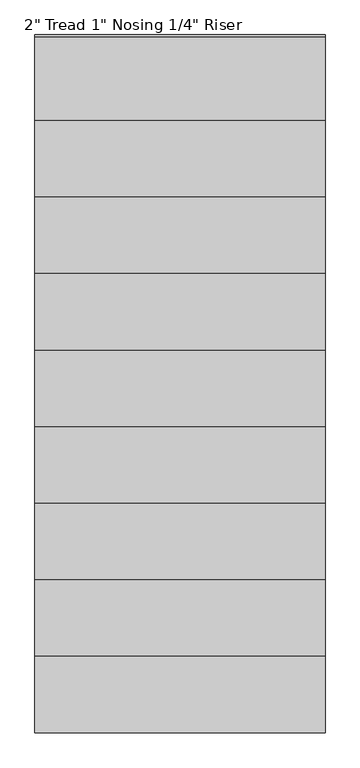
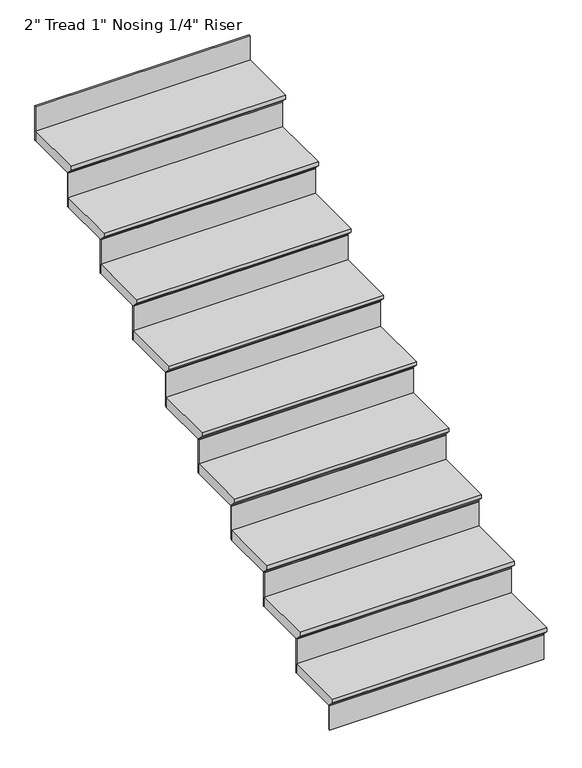
"""IFC4 building model written with IfcOpenShell, lengths in millimetres: stair flight geometry."""

from ifc_helpers import new_model, si_unit, frame, origin, place, context, project, spatial, polyline, outline, extrude, source, transform, mapped, element, save


def stair_flight_2c35b375(model_context):
    return source(origin(), model_context, "Body", "SweptSolid", [
        extrude(outline(polyline([(14615.2721081, -3378.2), (14920.0721081, -3378.2), (14920.0721081, -3429.0), (14640.6721081, -3429.0), (14640.6721081, -3422.65), (14615.2721081, -3397.25), (14615.2721081, -3378.2)])), frame((-263.7545099, 0.0, 0.0), z_axis=(1.0, 0.0, 0.0), x_axis=(0.0, 1.0, 0.0)), (0.0, 0.0, 1.0), 1058.3356324),
        extrude(outline(polyline([(794.5811225, 14647.0221081), (794.5811225, 14640.6721081), (-263.7545099, 14640.6721081), (-263.7545099, 14647.0221081), (794.5811225, 14647.0221081)])), frame((0.0, 0.0, -3556.0), z_axis=(0.0, 0.0, 1.0), x_axis=(1.0, 0.0, 0.0)), (0.0, 0.0, 1.0), 127.0),
        extrude(outline(polyline([(794.5811225, 14926.4221081), (794.5811225, 14920.0721081), (-263.7545099, 14920.0721081), (-263.7545099, 14926.4221081), (794.5811225, 14926.4221081)])), frame((0.0, 0.0, -3429.0), z_axis=(0.0, 0.0, 1.0), x_axis=(1.0, 0.0, 0.0)), (0.0, 0.0, 1.0), 177.8),
        extrude(outline(polyline([(14894.6721081, -3200.4), (15199.4721081, -3200.4), (15199.4721081, -3251.2), (14920.0721081, -3251.2), (14920.0721081, -3244.85), (14894.6721081, -3219.45), (14894.6721081, -3200.4)])), frame((-263.7545099, 0.0, 0.0), z_axis=(1.0, 0.0, 0.0), x_axis=(0.0, 1.0, 0.0)), (0.0, 0.0, 1.0), 1058.3356324),
        extrude(outline(polyline([(794.5811225, 15205.8221081), (794.5811225, 15199.4721081), (-263.7545099, 15199.4721081), (-263.7545099, 15205.8221081), (794.5811225, 15205.8221081)])), frame((0.0, 0.0, -3251.2), z_axis=(0.0, 0.0, 1.0), x_axis=(1.0, 0.0, 0.0)), (0.0, 0.0, 1.0), 177.8),
        extrude(outline(polyline([(15174.0721081, -3022.6), (15478.8721081, -3022.6), (15478.8721081, -3073.4), (15199.4721081, -3073.4), (15199.4721081, -3067.05), (15174.0721081, -3041.65), (15174.0721081, -3022.6)])), frame((-263.7545099, 0.0, 0.0), z_axis=(1.0, 0.0, 0.0), x_axis=(0.0, 1.0, 0.0)), (0.0, 0.0, 1.0), 1058.3356324),
        extrude(outline(polyline([(794.5811225, 15485.2221081), (794.5811225, 15478.8721081), (-263.7545099, 15478.8721081), (-263.7545099, 15485.2221081), (794.5811225, 15485.2221081)])), frame((0.0, 0.0, -3073.4), z_axis=(0.0, 0.0, 1.0), x_axis=(1.0, 0.0, 0.0)), (0.0, 0.0, 1.0), 177.8),
        extrude(outline(polyline([(15453.4721081, -2844.8), (15758.2721081, -2844.8), (15758.2721081, -2895.6), (15478.8721081, -2895.6), (15478.8721081, -2889.25), (15453.4721081, -2863.85), (15453.4721081, -2844.8)])), frame((-263.7545099, 0.0, 0.0), z_axis=(1.0, 0.0, 0.0), x_axis=(0.0, 1.0, 0.0)), (0.0, 0.0, 1.0), 1058.3356324),
        extrude(outline(polyline([(794.5811225, 15764.6221081), (794.5811225, 15758.2721081), (-263.7545099, 15758.2721081), (-263.7545099, 15764.6221081), (794.5811225, 15764.6221081)])), frame((0.0, 0.0, -2895.6), z_axis=(0.0, 0.0, 1.0), x_axis=(1.0, 0.0, 0.0)), (0.0, 0.0, 1.0), 177.8),
        extrude(outline(polyline([(15732.8721081, -2667.0), (16037.6721081, -2667.0), (16037.6721081, -2717.8), (15758.2721081, -2717.8), (15758.2721081, -2711.45), (15732.8721081, -2686.05), (15732.8721081, -2667.0)])), frame((-263.7545099, 0.0, 0.0), z_axis=(1.0, 0.0, 0.0), x_axis=(0.0, 1.0, 0.0)), (0.0, 0.0, 1.0), 1058.3356324),
        extrude(outline(polyline([(794.5811225, 16044.0221081), (794.5811225, 16037.6721081), (-263.7545099, 16037.6721081), (-263.7545099, 16044.0221081), (794.5811225, 16044.0221081)])), frame((0.0, 0.0, -2717.8), z_axis=(0.0, 0.0, 1.0), x_axis=(1.0, 0.0, 0.0)), (0.0, 0.0, 1.0), 177.8),
        extrude(outline(polyline([(16012.2721081, -2489.2), (16317.0721081, -2489.2), (16317.0721081, -2540.0), (16037.6721081, -2540.0), (16037.6721081, -2533.65), (16012.2721081, -2508.25), (16012.2721081, -2489.2)])), frame((-263.7545099, 0.0, 0.0), z_axis=(1.0, 0.0, 0.0), x_axis=(0.0, 1.0, 0.0)), (0.0, 0.0, 1.0), 1058.3356324),
        extrude(outline(polyline([(794.5811225, 16323.4221081), (794.5811225, 16317.0721081), (-263.7545099, 16317.0721081), (-263.7545099, 16323.4221081), (794.5811225, 16323.4221081)])), frame((0.0, 0.0, -2540.0), z_axis=(0.0, 0.0, 1.0), x_axis=(1.0, 0.0, 0.0)), (0.0, 0.0, 1.0), 177.8),
        extrude(outline(polyline([(16291.6721081, -2311.4), (16596.4721081, -2311.4), (16596.4721081, -2362.2), (16317.0721081, -2362.2), (16317.0721081, -2355.85), (16291.6721081, -2330.45), (16291.6721081, -2311.4)])), frame((-263.7545099, 0.0, 0.0), z_axis=(1.0, 0.0, 0.0), x_axis=(0.0, 1.0, 0.0)), (0.0, 0.0, 1.0), 1058.3356324),
        extrude(outline(polyline([(794.5811225, 16602.8221081), (794.5811225, 16596.4721081), (-263.7545099, 16596.4721081), (-263.7545099, 16602.8221081), (794.5811225, 16602.8221081)])), frame((0.0, 0.0, -2362.2), z_axis=(0.0, 0.0, 1.0), x_axis=(1.0, 0.0, 0.0)), (0.0, 0.0, 1.0), 177.8),
        extrude(outline(polyline([(16571.0721081, -2133.6), (16875.8721081, -2133.6), (16875.8721081, -2184.4), (16596.4721081, -2184.4), (16596.4721081, -2178.05), (16571.0721081, -2152.65), (16571.0721081, -2133.6)])), frame((-263.7545099, 0.0, 0.0), z_axis=(1.0, 0.0, 0.0), x_axis=(0.0, 1.0, 0.0)), (0.0, 0.0, 1.0), 1058.3356324),
        extrude(outline(polyline([(794.5811225, 16882.2221081), (794.5811225, 16875.8721081), (-263.7545099, 16875.8721081), (-263.7545099, 16882.2221081), (794.5811225, 16882.2221081)])), frame((0.0, 0.0, -2184.4), z_axis=(0.0, 0.0, 1.0), x_axis=(1.0, 0.0, 0.0)), (0.0, 0.0, 1.0), 177.8),
        extrude(outline(polyline([(794.5811225, 17161.6221081), (794.5811225, 17155.2721081), (-263.7545099, 17155.2721081), (-263.7545099, 17161.6221081), (794.5811225, 17161.6221081)])), frame((0.0, 0.0, -2006.6), z_axis=(0.0, 0.0, 1.0), x_axis=(1.0, 0.0, 0.0)), (0.0, 0.0, 1.0), 177.8),
        extrude(outline(polyline([(16850.4721081, -1955.8), (17155.2721081, -1955.8), (17155.2721081, -2006.6), (16875.8721081, -2006.6), (16875.8721081, -2000.25), (16850.4721081, -1974.85), (16850.4721081, -1955.8)])), frame((-263.7545099, 0.0, 0.0), z_axis=(1.0, 0.0, 0.0), x_axis=(0.0, 1.0, 0.0)), (0.0, 0.0, 1.0), 1058.3356324),
    ])


if __name__ == "__main__":
    model = new_model("IFC4")
    model_context = context("Model", 3, world=origin())
    ifc_project = project(units=[si_unit("LENGTHUNIT", "METRE", prefix="MILLI")], contexts=[model_context])
    site = spatial("IfcSite", under=ifc_project)
    building = spatial("IfcBuilding", under=site)
    placement = place(None, origin())
    stair_flight_shape = stair_flight_2c35b375(model_context)
    element("IfcStairFlight", 1, ObjectType="2\" Tread 1\" Nosing 1/4\" Riser", at=placement, inside=building, context=model_context, shape_type="MappedRepresentation", body=[
        mapped(stair_flight_shape, transform((0.0, 0.0, 0.0), x_axis=(1.0, 0.0, 0.0), y_axis=(0.0, 1.0, 0.0), z_axis=(0.0, 0.0, 1.0))),
    ])
    save(model, "model.ifc")

# Revit data of these elements
# Element 1 (IfcStairFlight, "2\" Tread 1\" Nosing 1/4\" Riser")
#   Materials on its faces: "Garpet - Sea Green"
# Materials
#   "Garpet - Sea Green": class "Carpet", colour RGB 107 175 109, transparency 0, Cost = 0
